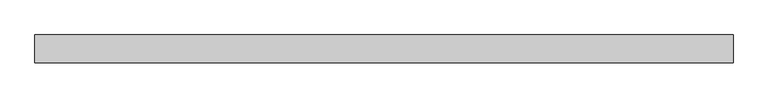
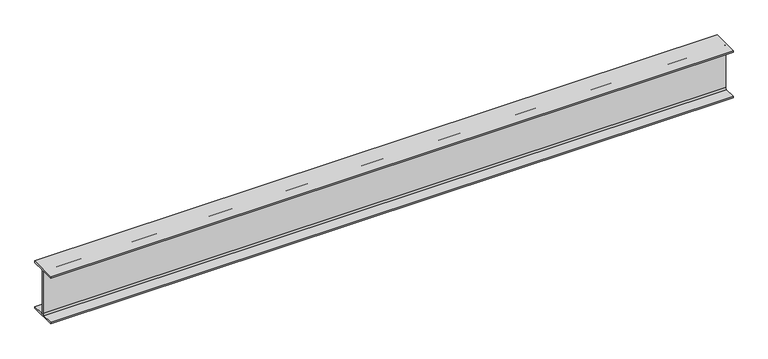
"""IFC4 building model written with IfcOpenShell, lengths in millimetres: beam geometry, Old_Steel Beam_H-KSD3502 : H_SB_ASB_H-250×125x6x9."""

from ifc_helpers import new_model, si_unit, point, frame, frame_2d, origin, place, context, project, spatial, polyline, circle_curve, trimmed, segment, composite_curve, outline, extrude, source, transform, mapped, element, save


def beam_31cb4085(model_context):
    return source(origin(), model_context, "Body", "SweptSolid", [
        extrude(outline(composite_curve([segment(polyline([(82.5, -141.5), (82.5, -151.7), (-82.5, -151.7), (-82.5, -141.5), (-11.9, -141.5)]), True, "CONTINUOUS"), segment(trimmed(circle_curve(frame_2d((-11.9, -132.6)), 8.9), [point((-11.9, -141.5))], [point((-3.0, -132.6))], True, "CARTESIAN"), True, "CONTINUOUS"), segment(polyline([(-3.0, -132.6), (-3.0, 132.6)]), True, "CONTINUOUS"), segment(trimmed(circle_curve(frame_2d((-11.9, 132.6)), 8.9), [point((-3.0, 132.6))], [point((-11.9, 141.5))], True, "CARTESIAN"), True, "CONTINUOUS"), segment(polyline([(-11.9, 141.5), (-82.5, 141.5), (-82.5, 151.7), (82.5, 151.7), (82.5, 141.5), (11.9, 141.5)]), True, "CONTINUOUS"), segment(trimmed(circle_curve(frame_2d((11.9, 132.6)), 8.9), [point((11.9, 141.5))], [point((3.0, 132.6))], True, "CARTESIAN"), True, "CONTINUOUS"), segment(polyline([(3.0, 132.6), (3.0, -132.6)]), True, "CONTINUOUS"), segment(trimmed(circle_curve(frame_2d((11.9, -132.6)), 8.9), [point((3.0, -132.6))], [point((11.9, -141.5))], True, "CARTESIAN"), True, "CONTINUOUS"), segment(polyline([(11.9, -141.5), (82.5, -141.5)]), True, "CONTINUOUS")], self_intersect=False)), frame((-2112.2999994, 0.0, 0.0), z_axis=(1.0, 0.0, 0.0), x_axis=(0.0, 1.0, 0.0)), (0.0, 0.0, 1.0), 4142.0999994),
    ])


if __name__ == "__main__":
    model = new_model("IFC4")
    model_context = context("Model", 3, world=origin())
    ifc_project = project(units=[si_unit("LENGTHUNIT", "METRE", prefix="MILLI")], contexts=[model_context])
    site = spatial("IfcSite", under=ifc_project)
    building = spatial("IfcBuilding", under=site)
    placement = place(None, origin())
    beam_shape = beam_31cb4085(model_context)
    element("IfcBeam", 1, ObjectType="Old_Steel Beam_H-KSD3502 : H_SB_ASB_H-250×125x6x9", at=placement, inside=building, context=model_context, shape_type="MappedRepresentation", body=[
        mapped(beam_shape, transform((0.0, 0.0, 0.0), x_axis=(1.0, 0.0, 0.0), y_axis=(0.0, 1.0, 0.0), z_axis=(0.0, 0.0, 1.0))),
    ])
    save(model, "model.ifc")

# Revit data of these elements
# Type "Old_Steel Beam_H-KSD3502 : H_SB_ASB_H-250×125x6x9"
#   Width = 12.5 cm
#   Web Thickness = 0.6 cm
#   Web Fillet = 1.2 cm
#   Warping Constant = 42539.8 cm⁶
#   Torsional Moment of Inertia = 7.8102 cm⁴
#   Torsional Modulus = 1.0 cm³
#   Section Area = 37.66 cm²
#   Plastic Modulus weak axis = 73.1 cm³
#   Plastic Modulus strong axis = 366.0 cm³
#   Perimeter = 0.97 m²/m
#   Nominal Weight = 29.60 kgf/m
#   Moment of Inertia weak axis = 294.00 cm⁴
#   Moment of Inertia strong axis = 4050.00 cm⁴
#   Height = 25.0 cm
#   Flange Thickness = 0.9 cm
#   Elastic Modulus weak axis = 47.0 cm³
#   Elastic Modulus strong axis = 324.0 cm³
#   Centroid Vertical = 12.5 cm
#   Centroid Horizontal = 6.25 cm
#   Length [instance default] = 1.5240 m
#   Structural Material [instance default] = Steel, 45-345
#   Assembly Code = ""
# Element 1 (IfcBeam, "Old_Steel Beam_H-KSD3502 : H_SB_ASB_H-250×125x6x9")
#   Structural Material = none
# Materials
#   "Steel, 45-345": class "Metal", colour RGB 189 187 185, transparency 0, Description = "Steel 345 MPa", Cost = 0
